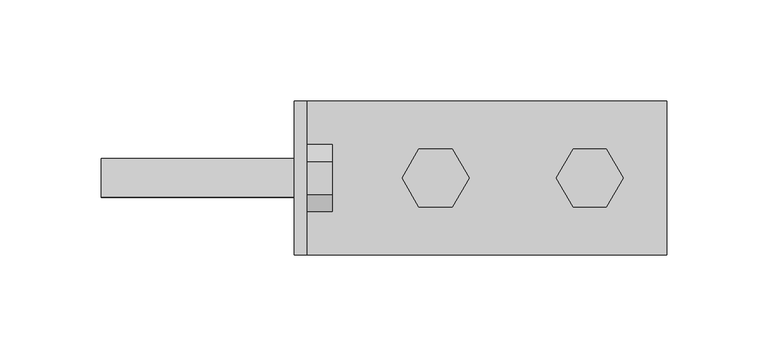
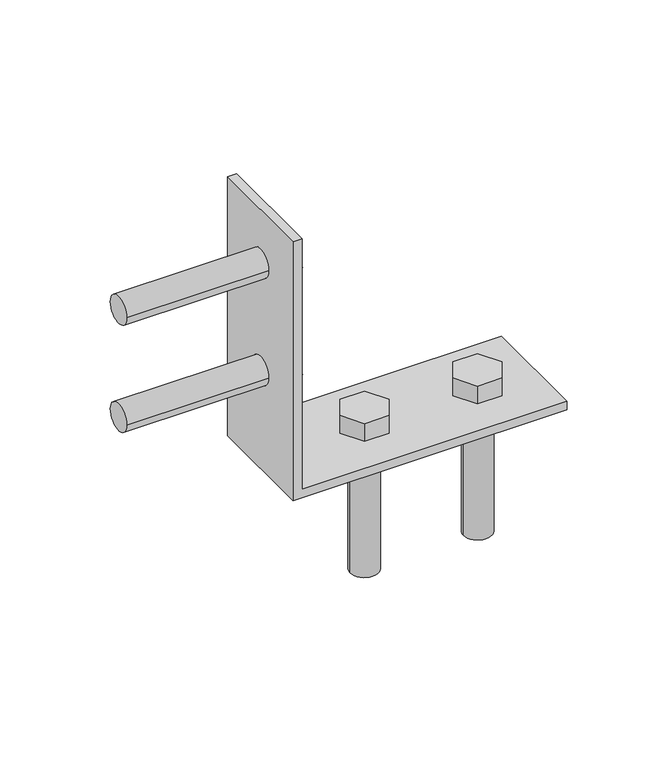
"""IFC4 building model written with IfcOpenShell, lengths in millimetres: fastener geometry, SIMPSON - HLPC/HLGPC Heavy Angles and Gussets : SIMPSON -HL73 - 3 X 7.25 - .75 Bolt - HDG."""

from ifc_helpers import new_model, si_unit, point, frame, frame_2d, origin, place, context, project, spatial, polyline, circle_curve, trimmed, segment, composite_curve, outline, extrude, source, transform, mapped, element, save
from ifc_brep_helpers import plane_surface, revolved_surface, advanced_brep


def fastener_2b3ee341(model_context):
    return source(origin(), model_context, "Body", "SolidModel", [
        extrude(outline(composite_curve([segment(trimmed(circle_curve(frame_2d((0.0, 69.85)), 9.525), [point((-9.525, 69.85))], [point((9.525, 69.85))], False, "CARTESIAN"), True, "CONTINUOUS"), segment(trimmed(circle_curve(frame_2d((0.0, 69.85)), 9.525), [point((9.525, 69.85))], [point((-9.525, 69.85))], False, "CARTESIAN"), True, "CONTINUOUS")], self_intersect=False)), frame((-95.5476562, 0.0, 0.0), z_axis=(1.0, 0.0, 0.0), x_axis=(0.0, 1.0, 0.0)), (0.0, 0.0, 1.0), 101.6),
        extrude(outline(polyline([(-16.4977839, 69.85), (-8.248892, 84.1375), (8.248892, 84.1375), (16.4977839, 69.85), (8.248892, 55.5625), (-8.248892, 55.5625), (-16.4977839, 69.85)])), frame((6.0523438, 0.0, 0.0), z_axis=(1.0, 0.0, 0.0), x_axis=(0.0, 1.0, 0.0)), (0.0, 0.0, 1.0), 12.7),
        extrude(outline(composite_curve([segment(trimmed(circle_curve(frame_2d((0.0, 146.05)), 9.525), [point((-9.525, 146.05))], [point((9.525, 146.05))], False, "CARTESIAN"), True, "CONTINUOUS"), segment(trimmed(circle_curve(frame_2d((0.0, 146.05)), 9.525), [point((9.525, 146.05))], [point((-9.525, 146.05))], False, "CARTESIAN"), True, "CONTINUOUS")], self_intersect=False)), frame((-95.5476562, 0.0, 0.0), z_axis=(1.0, 0.0, 0.0), x_axis=(0.0, 1.0, 0.0)), (0.0, 0.0, 1.0), 101.6),
        extrude(outline(polyline([(-16.4977839, 146.05), (-8.248892, 160.3375), (8.248892, 160.3375), (16.4977839, 146.05), (8.248892, 131.7625), (-8.248892, 131.7625), (-16.4977839, 146.05)])), frame((6.0523438, 0.0, 0.0), z_axis=(1.0, 0.0, 0.0), x_axis=(0.0, 1.0, 0.0)), (0.0, 0.0, 1.0), 12.7),
        extrude(outline(composite_curve([segment(trimmed(circle_curve(frame_2d((146.05, 0.0)), 9.525), [point((136.525, 0.0))], [point((155.575, 0.0))], False, "CARTESIAN"), True, "CONTINUOUS"), segment(trimmed(circle_curve(frame_2d((146.05, 0.0)), 9.525), [point((155.575, 0.0))], [point((136.525, 0.0))], False, "CARTESIAN"), True, "CONTINUOUS")], self_intersect=False)), frame((0.0, 0.0, -95.5476563), z_axis=(0.0, 0.0, 1.0), x_axis=(1.0, 0.0, 0.0)), (0.0, 0.0, 1.0), 101.6),
        extrude(outline(polyline([(129.5522161, 0.0), (137.801108, 14.2875), (154.298892, 14.2875), (162.5477839, 0.0), (154.298892, -14.2875), (137.801108, -14.2875), (129.5522161, 0.0)])), frame((0.0, 0.0, 6.0523437), z_axis=(0.0, 0.0, 1.0), x_axis=(1.0, 0.0, 0.0)), (0.0, 0.0, 1.0), 12.7),
        extrude(outline(composite_curve([segment(trimmed(circle_curve(frame_2d((69.85, 0.0)), 9.525), [point((60.325, 0.0))], [point((79.375, 0.0))], False, "CARTESIAN"), True, "CONTINUOUS"), segment(trimmed(circle_curve(frame_2d((69.85, 0.0)), 9.525), [point((79.375, 0.0))], [point((60.325, 0.0))], False, "CARTESIAN"), True, "CONTINUOUS")], self_intersect=False)), frame((0.0, 0.0, -95.5476563), z_axis=(0.0, 0.0, 1.0), x_axis=(1.0, 0.0, 0.0)), (0.0, 0.0, 1.0), 101.6),
        extrude(outline(polyline([(53.3522161, 0.0), (61.601108, 14.2875), (78.098892, 14.2875), (86.3477839, 0.0), (78.098892, -14.2875), (61.601108, -14.2875), (53.3522161, 0.0)])), frame((0.0, 0.0, 6.0523437), z_axis=(0.0, 0.0, 1.0), x_axis=(1.0, 0.0, 0.0)), (0.0, 0.0, 1.0), 12.7),
        advanced_brep(
        [(6.0523438, 38.1, 184.15), (6.0523438, -38.1, 184.15), (6.0523438, -38.1, 6.0523437), (6.0523438, 38.1, 6.0523437), (6.0523438, 9.525, 69.85), (6.0523438, -9.525, 69.85), (6.0523438, 9.525, 146.05), (6.0523438, -9.525, 146.05), (0.0, -38.1, 184.15), (0.0, 38.1, 184.15), (0.0, 38.1, 0.0), (0.0, -38.1, 0.0), (0.0, -9.525, 69.85), (0.0, 9.525, 69.85), (0.0, -9.525, 146.05), (0.0, 9.525, 146.05), (184.15, -38.1, 0.0), (184.15, -38.1, 6.0523437), (184.15, 38.1, 6.0523437), (184.15, 38.1, 0.0), (79.375, 0.0, 6.0523437), (60.325, 0.0, 6.0523437), (155.575, 0.0, 6.0523437), (136.525, 0.0, 6.0523437), (60.325, 0.0, 0.0), (79.375, 0.0, 0.0), (136.525, 0.0, 0.0), (155.575, 0.0, 0.0)],
        [
            (0, 1),
            (1, 2),
            (2, 3),
            (3, 0),
            (4, 5, circle_curve(frame((6.0523438, 0.0, 69.85), z_axis=(-1.0, 0.0, 0.0), x_axis=(0.0, 1.0, 0.0)), 9.525)),
            (5, 4, circle_curve(frame((6.0523438, 0.0, 69.85), z_axis=(-1.0, 0.0, 0.0), x_axis=(0.0, 1.0, 0.0)), 9.525)),
            (6, 7, circle_curve(frame((6.0523438, 0.0, 146.05), z_axis=(-1.0, 0.0, 0.0), x_axis=(0.0, 1.0, 0.0)), 9.525)),
            (7, 6, circle_curve(frame((6.0523438, 0.0, 146.05), z_axis=(-1.0, 0.0, 0.0), x_axis=(0.0, 1.0, 0.0)), 9.525)),
            (8, 9),
            (9, 10),
            (10, 11),
            (11, 8),
            (12, 13, circle_curve(frame((0.0, 0.0, 69.85), z_axis=(1.0, 0.0, 0.0), x_axis=(0.0, 1.0, 0.0)), 9.525)),
            (13, 12, circle_curve(frame((0.0, 0.0, 69.85), z_axis=(1.0, 0.0, 0.0), x_axis=(0.0, 1.0, 0.0)), 9.525)),
            (14, 15, circle_curve(frame((0.0, 0.0, 146.05), z_axis=(1.0, 0.0, 0.0), x_axis=(0.0, 1.0, 0.0)), 9.525)),
            (15, 14, circle_curve(frame((0.0, 0.0, 146.05), z_axis=(1.0, 0.0, 0.0), x_axis=(0.0, 1.0, 0.0)), 9.525)),
            (0, 9),
            (8, 1),
            (11, 16),
            (16, 17),
            (17, 2),
            (3, 18),
            (18, 19),
            (19, 10),
            (17, 18),
            (20, 21, circle_curve(frame((69.85, 0.0, 6.0523437), z_axis=(0.0, 0.0, -1.0), x_axis=(1.0, 0.0, 0.0)), 9.525)),
            (21, 20, circle_curve(frame((69.85, 0.0, 6.0523437), z_axis=(0.0, 0.0, -1.0), x_axis=(1.0, 0.0, 0.0)), 9.525)),
            (22, 23, circle_curve(frame((146.05, 0.0, 6.0523437), z_axis=(0.0, 0.0, -1.0), x_axis=(1.0, 0.0, 0.0)), 9.525)),
            (23, 22, circle_curve(frame((146.05, 0.0, 6.0523437), z_axis=(0.0, 0.0, -1.0), x_axis=(1.0, 0.0, 0.0)), 9.525)),
            (19, 16),
            (24, 25, circle_curve(frame((69.85, 0.0, 0.0), z_axis=(0.0, 0.0, 1.0), x_axis=(1.0, 0.0, 0.0)), 9.525)),
            (25, 24, circle_curve(frame((69.85, 0.0, 0.0), z_axis=(0.0, 0.0, 1.0), x_axis=(1.0, 0.0, 0.0)), 9.525)),
            (26, 27, circle_curve(frame((146.05, 0.0, 0.0), z_axis=(0.0, 0.0, 1.0), x_axis=(1.0, 0.0, 0.0)), 9.525)),
            (27, 26, circle_curve(frame((146.05, 0.0, 0.0), z_axis=(0.0, 0.0, 1.0), x_axis=(1.0, 0.0, 0.0)), 9.525)),
            (20, 25),
            (24, 21),
            (22, 27),
            (26, 23),
            (4, 13),
            (12, 5),
            (6, 15),
            (14, 7),
        ],
        [
            plane_surface(frame((6.0523438, -38.1, 184.15), z_axis=(1.0, 0.0, 0.0), x_axis=(0.0, -1.0, 0.0))),
            plane_surface(frame((0.0, -38.1, 184.15), z_axis=(-1.0, 0.0, 0.0), x_axis=(0.0, 1.0, 0.0))),
            plane_surface(frame((6.0523438, 38.1, 184.15), z_axis=(0.0, 0.0, 1.0), x_axis=(-1.0, 0.0, 0.0))),
            plane_surface(frame((6.0523438, -38.1, 184.15), z_axis=(0.0, -1.0, 0.0), x_axis=(-1.0, 0.0, 0.0))),
            plane_surface(frame((6.0523438, 38.1, 6.0523437), z_axis=(0.0, 1.0, 0.0), x_axis=(-1.0, 0.0, 0.0))),
            plane_surface(frame((0.0, 38.1, 6.0523437), z_axis=(0.0, 0.0, 1.0), x_axis=(-1.0, 0.0, 0.0))),
            plane_surface(frame((0.0, 38.1, 0.0), z_axis=(0.0, 0.0, -1.0), x_axis=(1.0, 0.0, 0.0))),
            plane_surface(frame((184.15, -38.1, 6.0523437), z_axis=(1.0, 0.0, 0.0), x_axis=(0.0, 0.0, -1.0))),
            revolved_surface(polyline([(79.375, 0.0, 6.0523437), (79.375, 0.0, 0.0)]), (69.85, 0.0, 0.0), (0.0, 0.0, 1.0)),
            revolved_surface(polyline([(155.57500000000002, 0.0, 6.0523437), (155.57500000000002, 0.0, 0.0)]), (146.05, 0.0, 0.0), (0.0, 0.0, 1.0)),
            revolved_surface(polyline([(6.0523438, 9.525, 69.85), (0.0, 9.525, 69.85)]), (0.0, 0.0, 69.85), (1.0, 0.0, 0.0)),
            revolved_surface(polyline([(6.0523438, 9.525, 146.05), (0.0, 9.525, 146.05)]), (0.0, 0.0, 146.05), (1.0, 0.0, 0.0)),
        ],
        [
            (0, [[1, 2, 3, 4], [5, 6], [7, 8]]),
            (1, [[9, 10, 11, 12], [13, 14], [15, 16]]),
            (2, [[-1, 17, -9, 18]]),
            (3, [[-2, -18, -12, 19, 20, 21]]),
            (4, [[-4, 22, 23, 24, -10, -17]]),
            (5, [[25, -22, -3, -21], [26, 27], [28, 29]]),
            (6, [[30, -19, -11, -24], [31, 32], [33, 34]]),
            (7, [[-25, -20, -30, -23]]),
            (8, [[35, -31, 36, -26]]),
            (8, [[-35, -27, -36, -32]]),
            (9, [[37, -33, 38, -28]]),
            (9, [[-37, -29, -38, -34]]),
            (10, [[39, -13, 40, -5]]),
            (10, [[-39, -6, -40, -14]]),
            (11, [[41, -15, 42, -7]]),
            (11, [[-41, -8, -42, -16]]),
        ],
    ),
    ])


if __name__ == "__main__":
    model = new_model("IFC4")
    model_context = context("Model", 3, world=origin())
    ifc_project = project(units=[si_unit("LENGTHUNIT", "METRE", prefix="MILLI")], contexts=[model_context])
    site = spatial("IfcSite", under=ifc_project)
    building = spatial("IfcBuilding", under=site)
    placement = place(None, origin())
    fastener_shape = fastener_2b3ee341(model_context)
    element("IfcFastener", 1, ObjectType="SIMPSON - HLPC/HLGPC Heavy Angles and Gussets : SIMPSON -HL73 - 3 X 7.25 - .75 Bolt - HDG", at=placement, inside=building, context=model_context, shape_type="MappedRepresentation", body=[
        mapped(fastener_shape, transform((0.0, 0.0, 0.0), x_axis=(1.0, 0.0, 0.0), y_axis=(0.0, 1.0, 0.0), z_axis=(0.0, 0.0, 1.0))),
    ])
    save(model, "model.ifc")

# Revit data of these elements
# Type "SIMPSON - HLPC/HLGPC Heavy Angles and Gussets : SIMPSON -HL73 - 3 X 7.25 - .75 Bolt - HDG"
#   URL = "https://www.strongtie.com/classiccollection_architecturalproductsgroup/hlpc-hlgpc_productgroup_wcc/p/hlpc.hlgpc"
#   L = 0' - 3"
#   Hole Radius = 0' - 0 3/8"
#   D4 = 0' - 3"
#   D2 = 0' - 5"
#   D1 = 0' - 1 1/2"
#   D3 = 0' - 2 3/4"
#   Ga. = 0' - 0 61/256"
#   W1 & W2 = 0' - 7 1/4"
#   Default Elevation = 4' - 0"
#   Bolt Visibility - 3B = no
#   Bolt Visibility - 3A = no
#   Bolt Visibility - 2B = no
#   Bolt Visibility - 2A = no
#   Bolt Visibility - 1B = yes
#   Bolt Visibility - 1A = yes
#   Bolt Visibility = yes
#   Bolt Size = element 1298415
# Element 1 (IfcFastener, "SIMPSON - HLPC/HLGPC Heavy Angles and Gussets : SIMPSON -HL73 - 3 X 7.25 - .75 Bolt - HDG")
#   Materials on its faces: "1\" GALV. LAG BOLT (LENGTH = 1/2\" SHY OF GLULAM DEPTH) -  (GALV. THRU BOLT IF PLATE ON OPP. SIDE OF STRUCT MEMBER)"
# Materials
#   "1\" GALV. LAG BOLT (LENGTH = 1/2\" SHY OF GLULAM DEPTH) -  (GALV. THRU BOLT IF PLATE ON OPP. SIDE OF STRUCT MEMBER)": class "Generic", colour RGB 120 120 120, transparency 0, Cost = 0
